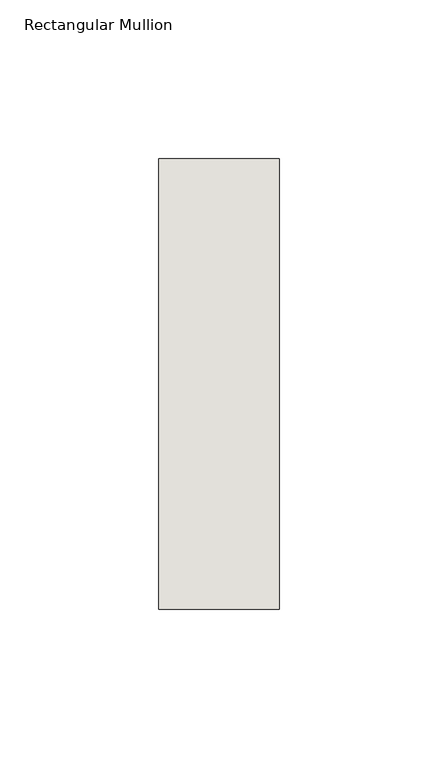
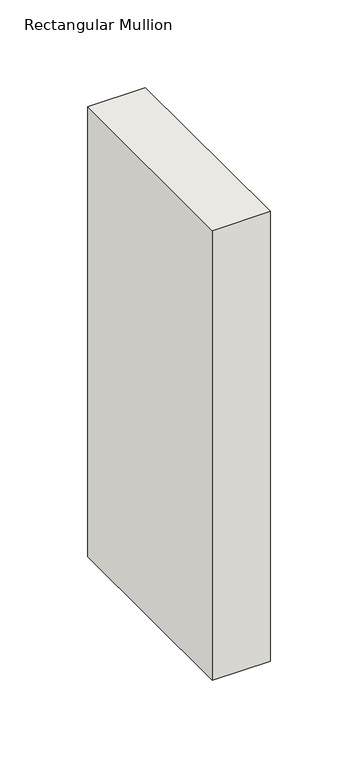
"""IFC4 building model written with IfcOpenShell, lengths in millimetres: wall geometry, Rectangular Mullion : NLRS_21_CWM_hsb-regel 38x142_gen_rsf."""

from ifc_helpers import new_model, si_unit, frame, origin, place, context, project, spatial, polyline, outline, extrude, source, transform, mapped, element, save


def rectangular_mullion_6d68dd6a(model_context):
    return source(origin(), model_context, "Body", "SweptSolid", [
        extrude(outline(polyline([(0.0, -71.0), (-38.0, -71.0), (-38.0, 71.0), (0.0, 71.0), (0.0, -71.0)])), frame((0.0, 0.0, -312.8441061), z_axis=(0.0, 0.0, 1.0), x_axis=(1.0, 0.0, 0.0)), (0.0, 0.0, 1.0), 312.8441061),
    ])


if __name__ == "__main__":
    model = new_model("IFC4")
    model_context = context("Model", 3, world=origin())
    ifc_project = project(units=[si_unit("LENGTHUNIT", "METRE", prefix="MILLI")], contexts=[model_context])
    site = spatial("IfcSite", under=ifc_project)
    building = spatial("IfcBuilding", under=site)
    placement = place(None, origin())
    rectangular_mullion_shape = rectangular_mullion_6d68dd6a(model_context)
    element("IfcWall", 1, ObjectType="Rectangular Mullion : NLRS_21_CWM_hsb-regel 38x142_gen_rsf", at=placement, inside=building, context=model_context, shape_type="MappedRepresentation", body=[
        mapped(rectangular_mullion_shape, transform((0.0, 0.0, 0.0), x_axis=(1.0, 0.0, 0.0), y_axis=(0.0, 1.0, 0.0), z_axis=(0.0, 0.0, 1.0))),
    ])
    save(model, "model.ifc")

# Revit data of these elements
# Type "Rectangular Mullion : NLRS_21_CWM_hsb-regel 38x142_gen_rsf"
#   Type IfcGUID = "07M7mRoiH1CR8m_RSKIwpF"
#   Assembly Code = "21.10"
#   IfcExportAs = "IfcWall"
#   built-in parameter 1007322 = 0.465879 (stored number, unit not read)
#   built-in parameter 1007321 = 0.062336 (stored number, unit not read)
#   built-in parameter 1007320 = 0.062336 (stored number, unit not read)
# Element 1 (IfcWall, "Rectangular Mullion : NLRS_21_CWM_hsb-regel 38x142_gen_rsf")
#   Materials on its faces: "NLRS_i2_hout naaldhout vuren_gen_rsf"
# Materials
#   "NLRS_i2_hout naaldhout vuren_gen_rsf": class "I - Hout", colour RGB 234 199 147, transparency 0, Keynote = "i2", Manufacturer = "Revit Standards Foundation", URL = "www.revitstandards.org", Description = "hout vuren", Cost = 0
